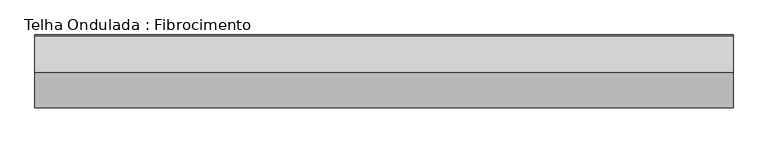
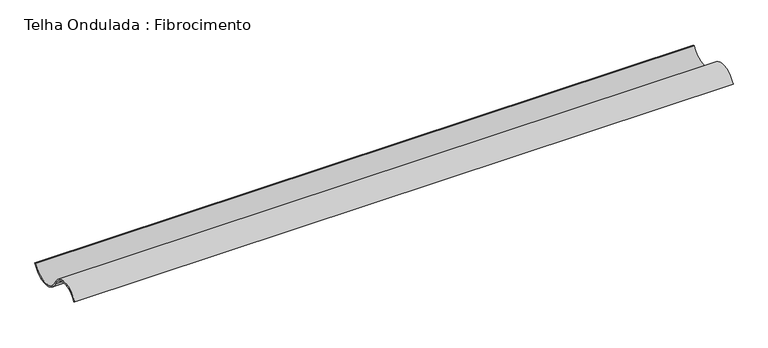
"""IFC4 building model written with IfcOpenShell, lengths in millimetres: beam geometry, Telha Ondulada : Fibrocimento."""

from ifc_helpers import new_model, si_unit, point, frame, frame_2d, origin, place, context, project, spatial, polyline, circle_curve, trimmed, segment, composite_curve, outline, extrude, source, transform, mapped, element, save


def telha_ondulada_fibrocimento_25135e7b(model_context):
    return source(origin(), model_context, "Body", "SweptSolid", [
        extrude(outline(composite_curve([segment(trimmed(circle_curve(frame_2d((68.3970135, 71.7939461)), 66.7939461), [point((8.3970135, 42.4437972))], [point((128.3970135, 42.4437972))], True, "CARTESIAN"), True, "CONTINUOUS"), segment(polyline([(128.3970135, 42.4437972), (132.8884385, 40.2467307)]), True, "CONTINUOUS"), segment(trimmed(circle_curve(frame_2d((68.3970135, 71.7939461)), 71.7939461), [point((132.8884385, 40.2467307))], [point((3.9055884, 40.2467307))], False, "CARTESIAN"), True, "CONTINUOUS"), segment(trimmed(circle_curve(frame_2d((-51.6029865, 13.0936483)), 61.7939461), [point((3.9055884, 40.2467307))], [point((-107.1115615, 40.2467307))], True, "CARTESIAN"), True, "CONTINUOUS"), segment(polyline([(-107.1115615, 40.2467307), (-111.6029865, 42.4437972)]), True, "CONTINUOUS"), segment(trimmed(circle_curve(frame_2d((-51.6029865, 13.0936483)), 66.7939461), [point((-111.6029865, 42.4437972))], [point((8.3970135, 42.4437972))], False, "CARTESIAN"), True, "CONTINUOUS")], self_intersect=False)), frame((-1169.5561442, 0.0, 0.0), z_axis=(1.0, 0.0, 0.0), x_axis=(0.0, 1.0, 0.0)), (0.0, 0.0, 1.0), 2339.1122884),
    ])


if __name__ == "__main__":
    model = new_model("IFC4")
    model_context = context("Model", 3, world=origin())
    ifc_project = project(units=[si_unit("LENGTHUNIT", "METRE", prefix="MILLI")], contexts=[model_context])
    site = spatial("IfcSite", under=ifc_project)
    building = spatial("IfcBuilding", under=site)
    placement = place(None, origin())
    telha_ondulada_fibrocimento_shape = telha_ondulada_fibrocimento_25135e7b(model_context)
    element("IfcBeam", 1, ObjectType="Telha Ondulada : Fibrocimento", at=placement, inside=building, context=model_context, shape_type="MappedRepresentation", body=[
        mapped(telha_ondulada_fibrocimento_shape, transform((0.0, 0.0, 0.0), x_axis=(1.0, 0.0, 0.0), y_axis=(0.0, 1.0, 0.0), z_axis=(0.0, 0.0, 1.0))),
    ])
    save(model, "model.ifc")

# Revit data of these elements
# Type "Telha Ondulada : Fibrocimento"
#   Description = "TELHA ONDULADA FIBROCIMENTO"
#   Cost = 5
#   Length [instance default] = 1.524 m
#   b = 0.07 m
#   h = 0.16 m
#   Structural Material = .TELHA DE FIBROCIMENTO
#   Assembly Code = ""
# Element 1 (IfcBeam, "Telha Ondulada : Fibrocimento")
#   Materials on its faces: ".TELHA DE FIBROCIMENTO"
# Materials
#   ".TELHA DE FIBROCIMENTO": class "CC_TELHADO", colour RGB 77 77 76, transparency 0, Description = "TELHA ONDULADA FIBROCIMENTO", Cost = 0
